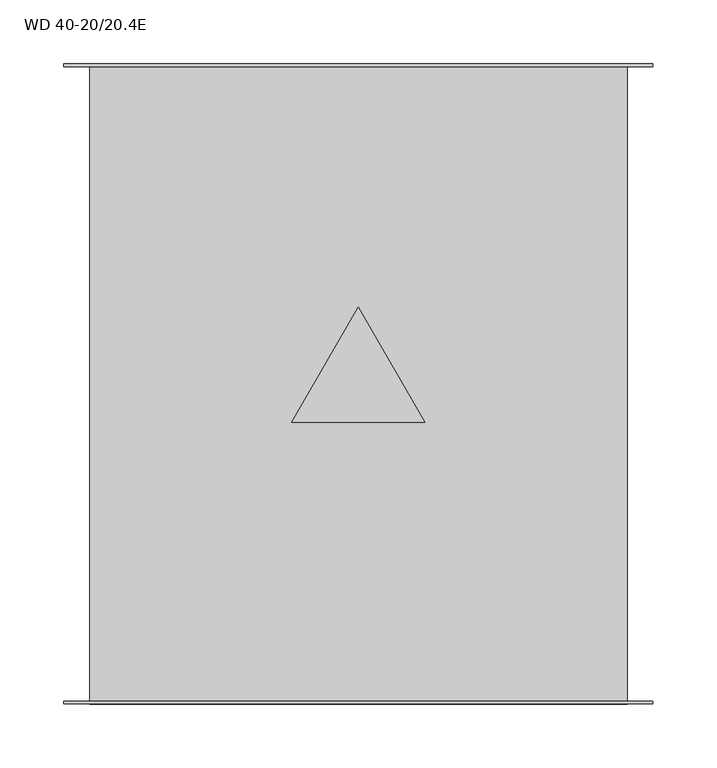
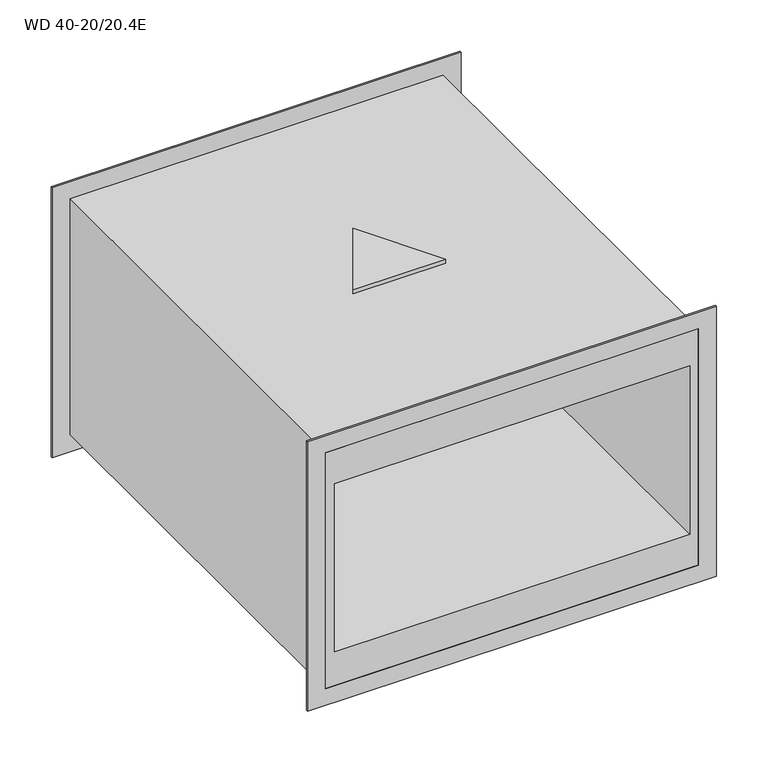
"""IFC4 building model written with IfcOpenShell, lengths in millimetres: proxy geometry, Вентилятор канальный WD (WDN) : WD 40-20/20.4E."""

from ifc_helpers import new_model, si_unit, frame, origin, place, context, project, spatial, polyline, outline, extrude, source, transform, mapped, element, save


def wd_40_20_20_4e_335ec504(model_context):
    return source(origin(), model_context, "Body", "SweptSolid", [
        extrude(outline(polyline([(-51.9615242, -30.0), (0.0, 60.0), (51.9615242, -30.0), (-51.9615242, -30.0)])), frame((0.0, 0.0, 140.5), z_axis=(0.0, 0.0, 1.0), x_axis=(1.0, 0.0, 0.0)), (0.0, 0.0, 1.0), 5.0),
        extrude(outline(polyline([(160.5, 230.0), (160.5, -230.0), (-160.5, -230.0), (-160.5, 230.0), (160.5, 230.0)]), holes=[polyline([(-140.5, 210.0), (-140.5, -210.0), (140.5, -210.0), (140.5, 210.0), (-140.5, 210.0)])]), frame((0.0, 248.0, 0.0), z_axis=(0.0, 1.0, 0.0), x_axis=(0.0, 0.0, 1.0)), (0.0, 0.0, 1.0), 2.0),
        extrude(outline(polyline([(160.5, -230.0), (-160.5, -230.0), (-160.5, 230.0), (160.5, 230.0), (160.5, -230.0)]), holes=[polyline([(140.5, 210.0), (-140.5, 210.0), (-140.5, -210.0), (140.5, -210.0), (140.5, 210.0)])]), frame((0.0, -250.0, 0.0), z_axis=(0.0, 1.0, 0.0), x_axis=(0.0, 0.0, 1.0)), (0.0, 0.0, 1.0), 2.0),
        extrude(outline(polyline([(140.5, 210.0), (140.5, -210.0), (-140.5, -210.0), (-140.5, 210.0), (140.5, 210.0)]), holes=[polyline([(100.0, 200.0), (-100.0, 200.0), (-100.0, -200.0), (100.0, -200.0), (100.0, 200.0)])]), frame((0.0, -250.0, 0.0), z_axis=(0.0, 1.0, 0.0), x_axis=(0.0, 0.0, 1.0)), (0.0, 0.0, 1.0), 500.0),
    ])


if __name__ == "__main__":
    model = new_model("IFC4")
    model_context = context("Model", 3, world=origin())
    ifc_project = project(units=[si_unit("LENGTHUNIT", "METRE", prefix="MILLI")], contexts=[model_context])
    site = spatial("IfcSite", under=ifc_project)
    building = spatial("IfcBuilding", under=site)
    placement = place(None, origin())
    wd_40_20_20_4e_shape = wd_40_20_20_4e_335ec504(model_context)
    element("IfcBuildingElementProxy", 1, Name="Вентилятор канальный WD (WDN) : WD 40-20/20.4E", ObjectType="Вентилятор канальный WD (WDN) : WD 40-20/20.4E", at=placement, inside=building, context=model_context, shape_type="MappedRepresentation", body=[
        mapped(wd_40_20_20_4e_shape, transform((0.0, 0.0, 0.0), x_axis=(1.0, 0.0, 0.0), y_axis=(0.0, 1.0, 0.0), z_axis=(0.0, 0.0, 1.0))),
    ])
    save(model, "model.ifc")

# Revit data of these elements
# Type "Вентилятор канальный WD (WDN) : WD 40-20/20.4E"
#   Manufacturer = "WAER"
#   URL = "https://waer-air.com/"
#   ADSK_Система_Имя [instance default] = ""
#   ADSK_Наименование краткое = "WD 40-20/20.4E"
#   ADSK_Наименование = "Венилятор канальный WD 40-20/20.4E"
#   ADSK_Масса_Текст = "14.4"
#   ADSK_Марка = ""
#   ADSK_Код изделия = ""
#   ADSK_Завод-изготовитель = "WAER"
#   ADSK_Единица измерения = "шт."
#   Ширина_Е = 420 mm
#   Высота_К = 281 mm
#   ADSK_Ток = 1.52 A
#   ADSK_Расход воздуха = 0 m³/h
#   ADSK_Размер_Ширина = 400 mm
#   ADSK_Размер_Длина = 500 mm
#   ADSK_Размер_Высота = 200 mm
#   ADSK_Потеря давления воздуха = 0.0 Pa
#   ADSK_Полная мощность = 334.4 VA
#   ADSK_Номинальная мощность = 0.33 W
#   ADSK_Напряжение = 220 V
#   ADSK_Масса = 14.4
#   ADSK_Количество = 1
#   ADSK_Количество фаз = 1
#   ADSK_Классификация нагрузок = ОВК
#   Default Elevation = 0
#   Keynote = ""
